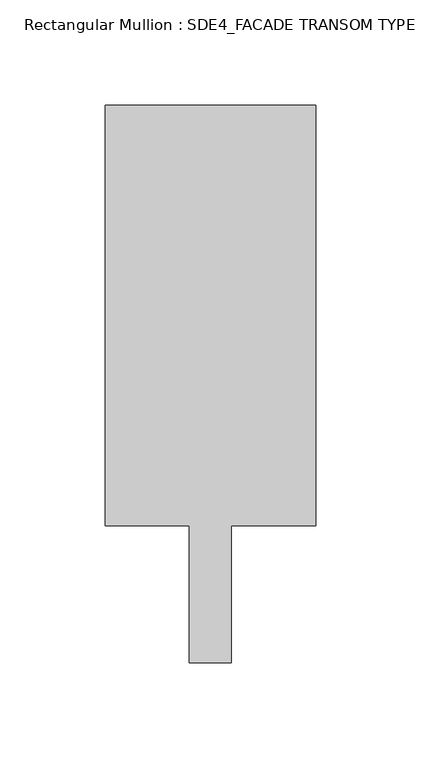
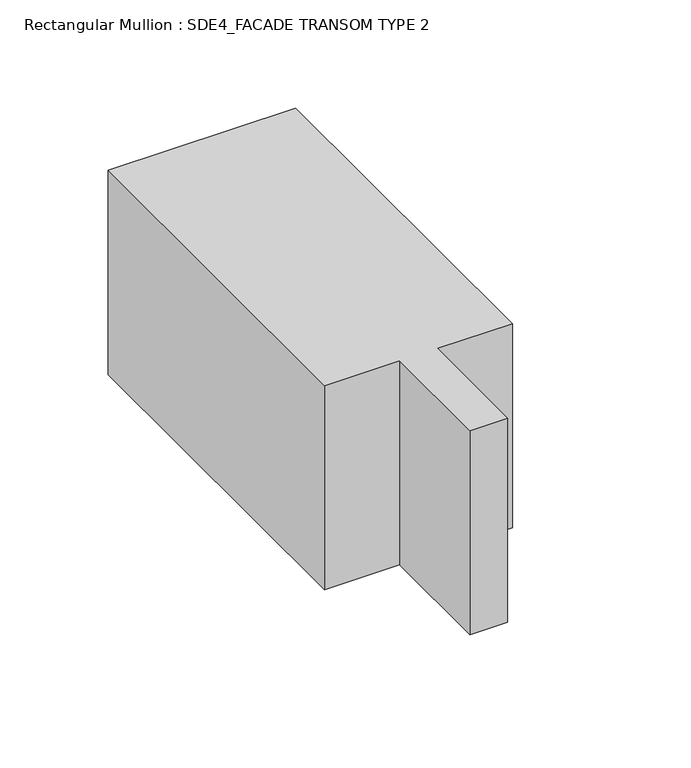
"""IFC4 building model written with IfcOpenShell, lengths in millimetres: member geometry, Rectangular Mullion : SDE4_FACADE TRANSOM TYPE 2."""

from ifc_helpers import new_model, si_unit, frame, origin, place, context, project, spatial, polyline, outline, extrude, source, transform, mapped, element, save


def rectangular_mullion_sde4_facade_transom_type_2_2e46f9e7(model_context):
    return source(origin(), model_context, "Body", "SweptSolid", [
        extrude(outline(polyline([(50.0, 132.5), (50.0, -67.5), (10.0, -67.5), (10.0, -132.5), (-10.0, -132.5), (-10.0, -67.5), (-50.0, -67.5), (-50.0, 132.5), (50.0, 132.5)])), frame((0.0, 0.0, -115.0), z_axis=(0.0, 0.0, 1.0), x_axis=(1.0, 0.0, 0.0)), (0.0, 0.0, 1.0), 115.0),
    ])


if __name__ == "__main__":
    model = new_model("IFC4")
    model_context = context("Model", 3, world=origin())
    ifc_project = project(units=[si_unit("LENGTHUNIT", "METRE", prefix="MILLI")], contexts=[model_context])
    site = spatial("IfcSite", under=ifc_project)
    building = spatial("IfcBuilding", under=site)
    placement = place(None, origin())
    rectangular_mullion_sde4_facade_transom_type_2_shape = rectangular_mullion_sde4_facade_transom_type_2_2e46f9e7(model_context)
    element("IfcMember", 1, ObjectType="Rectangular Mullion : SDE4_FACADE TRANSOM TYPE 2", at=placement, inside=building, context=model_context, shape_type="MappedRepresentation", body=[
        mapped(rectangular_mullion_sde4_facade_transom_type_2_shape, transform((0.0, 0.0, 0.0), x_axis=(1.0, 0.0, 0.0), y_axis=(0.0, 1.0, 0.0), z_axis=(0.0, 0.0, 1.0))),
    ])
    save(model, "model.ifc")

# Revit data of these elements
# Type "Rectangular Mullion : SDE4_FACADE TRANSOM TYPE 2"
#   built-in parameter 1007322 = 0.869423 (stored number, unit not read)
#   built-in parameter 1007321 = 0.164042 (stored number, unit not read)
#   built-in parameter 1007320 = 0.164042 (stored number, unit not read)
